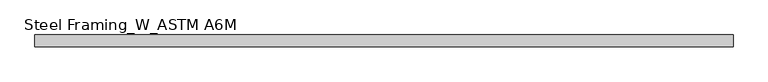
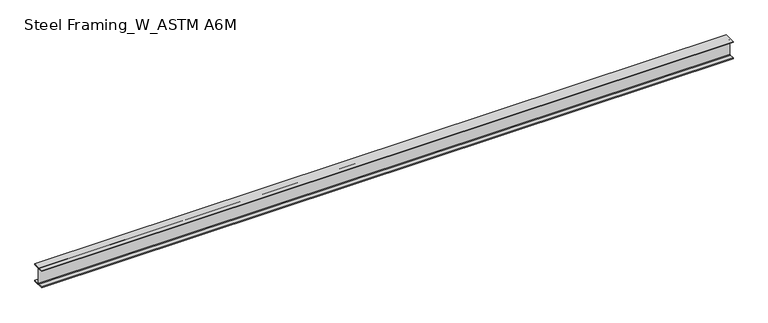
"""IFC4 building model written with IfcOpenShell, lengths in millimetres: beam geometry, Steel Framing_W_ASTM A6M : H_SB_AR_S02_W200x31.3_RB4."""

from ifc_helpers import new_model, si_unit, point, frame, frame_2d, origin, place, context, project, spatial, polyline, circle_curve, trimmed, segment, composite_curve, outline, extrude, source, transform, mapped, element, save


def steel_framing_w_astm_a6m_00f88cfe(model_context):
    return source(origin(), model_context, "Body", "SweptSolid", [
        extrude(outline(composite_curve([segment(polyline([(67.0, -94.8), (67.0, -105.0), (-67.0, -105.0), (-67.0, -94.8), (-10.775, -94.8)]), True, "CONTINUOUS"), segment(trimmed(circle_curve(frame_2d((-10.775, -87.2)), 7.6), [point((-10.775, -94.8))], [point((-3.175, -87.2))], True, "CARTESIAN"), True, "CONTINUOUS"), segment(polyline([(-3.175, -87.2), (-3.175, 87.2)]), True, "CONTINUOUS"), segment(trimmed(circle_curve(frame_2d((-10.775, 87.2)), 7.6), [point((-3.175, 87.2))], [point((-10.775, 94.8))], True, "CARTESIAN"), True, "CONTINUOUS"), segment(polyline([(-10.775, 94.8), (-67.0, 94.8), (-67.0, 105.0), (67.0, 105.0), (67.0, 94.8), (10.775, 94.8)]), True, "CONTINUOUS"), segment(trimmed(circle_curve(frame_2d((10.775, 87.2)), 7.6), [point((10.775, 94.8))], [point((3.175, 87.2))], True, "CARTESIAN"), True, "CONTINUOUS"), segment(polyline([(3.175, 87.2), (3.175, -87.2)]), True, "CONTINUOUS"), segment(trimmed(circle_curve(frame_2d((10.775, -87.2)), 7.6), [point((3.175, -87.2))], [point((10.775, -94.8))], True, "CARTESIAN"), True, "CONTINUOUS"), segment(polyline([(10.775, -94.8), (67.0, -94.8)]), True, "CONTINUOUS")], self_intersect=False)), frame((-3904.65, 0.0, 0.0), z_axis=(1.0, 0.0, 0.0), x_axis=(0.0, 1.0, 0.0)), (0.0, 0.0, 1.0), 7965.4),
    ])


if __name__ == "__main__":
    model = new_model("IFC4")
    model_context = context("Model", 3, world=origin())
    ifc_project = project(units=[si_unit("LENGTHUNIT", "METRE", prefix="MILLI")], contexts=[model_context])
    site = spatial("IfcSite", under=ifc_project)
    building = spatial("IfcBuilding", under=site)
    placement = place(None, origin())
    steel_framing_w_astm_a6m_shape = steel_framing_w_astm_a6m_00f88cfe(model_context)
    element("IfcBeam", 1, ObjectType="Steel Framing_W_ASTM A6M : H_SB_AR_S02_W200x31.3_RB4", at=placement, inside=building, context=model_context, shape_type="MappedRepresentation", body=[
        mapped(steel_framing_w_astm_a6m_shape, transform((0.0, 0.0, 0.0), x_axis=(1.0, 0.0, 0.0), y_axis=(0.0, 1.0, 0.0), z_axis=(0.0, 0.0, 1.0))),
    ])
    save(model, "model.ifc")

# Revit data of these elements
# Type "Steel Framing_W_ASTM A6M : H_SB_AR_S02_W200x31.3_RB4"
#   Type Mark = "RB4"
#   Section Name Key = "W8x21"
#   Width = 13.4 cm
#   Web Thickness = 0.635 cm
#   Web Fillet = 0.76 cm
#   Warping Constant = 40800.0 cm⁶
#   Torsional Moment of Inertia = 11.70 cm⁴
#   Section Area = 39.7 cm²
#   Plastic Modulus weak axis = 93.2 cm³
#   Plastic Modulus strong axis = 334.0 cm³
#   Perimeter = 0.93 m²/m
#   Nominal Weight = 31.30 kgf/m
#   Moment of Inertia weak axis = 407.00 cm⁴
#   Moment of Inertia strong axis = 3130.00 cm⁴
#   Height = 21.0 cm
#   Flange Thickness = 1.02 cm
#   Elastic Modulus weak axis = 60.8 cm³
#   Elastic Modulus strong axis = 298.0 cm³
#   Centroid Vertical = 10.5 cm
#   Centroid Horizontal = 6.7 cm
#   Length [instance default] = 1500 mm
#   Structural Material [instance default] = Steel, 45-345
#   Bolt Spacing = 0
#   Assembly Code = ""
# Element 1 (IfcBeam, "Steel Framing_W_ASTM A6M : H_SB_AR_S02_W200x31.3_RB4")
#   Materials on its faces: "Steel, 45-345"
# Materials
#   "Steel, 45-345": class "Metal", colour RGB 189 187 185, transparency 0, Description = "Steel 345 MPa", Cost = 0
